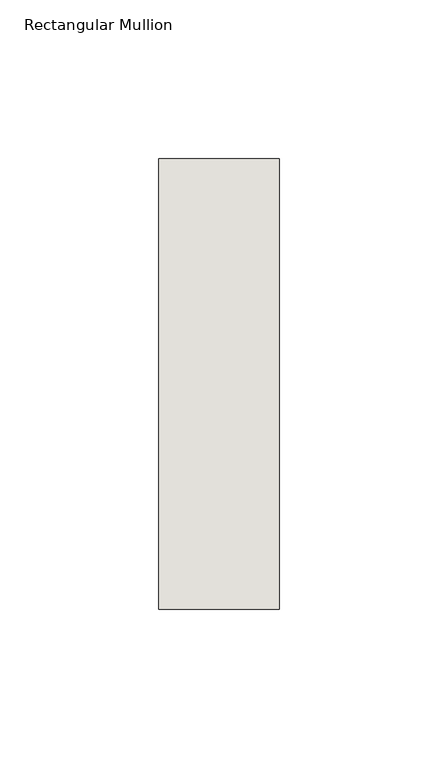
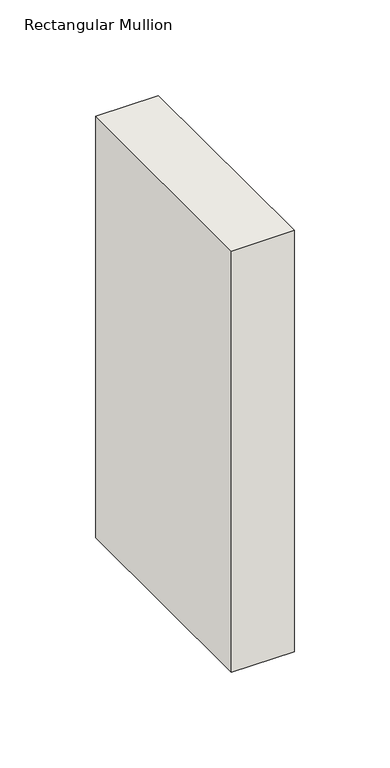
"""IFC4 building model written with IfcOpenShell, lengths in millimetres: wall geometry, Rectangular Mullion : NLRS_21_CWM_hsb-regel 38x142_gen_rsf."""

from ifc_helpers import new_model, si_unit, frame, origin, place, context, project, spatial, polyline, outline, extrude, source, transform, mapped, element, save


def rectangular_mullion_985b883b(model_context):
    return source(origin(), model_context, "Body", "SweptSolid", [
        extrude(outline(polyline([(-38.0, -71.0), (-38.0, 71.0), (0.0, 71.0), (0.0, -71.0), (-38.0, -71.0)])), frame((0.0, 0.0, -269.0000003), z_axis=(0.0, 0.0, 1.0), x_axis=(1.0, 0.0, 0.0)), (0.0, 0.0, 1.0), 269.0000003),
    ])


if __name__ == "__main__":
    model = new_model("IFC4")
    model_context = context("Model", 3, world=origin())
    ifc_project = project(units=[si_unit("LENGTHUNIT", "METRE", prefix="MILLI")], contexts=[model_context])
    site = spatial("IfcSite", under=ifc_project)
    building = spatial("IfcBuilding", under=site)
    placement = place(None, origin())
    rectangular_mullion_shape = rectangular_mullion_985b883b(model_context)
    element("IfcWall", 1, ObjectType="Rectangular Mullion : NLRS_21_CWM_hsb-regel 38x142_gen_rsf", at=placement, inside=building, context=model_context, shape_type="MappedRepresentation", body=[
        mapped(rectangular_mullion_shape, transform((0.0, 0.0, 0.0), x_axis=(1.0, 0.0, 0.0), y_axis=(0.0, 1.0, 0.0), z_axis=(0.0, 0.0, 1.0))),
    ])
    save(model, "model.ifc")

# Revit data of these elements
# Type "Rectangular Mullion : NLRS_21_CWM_hsb-regel 38x142_gen_rsf"
#   Type IfcGUID = "07M7mRoiH1CR8m_RSKIwpF"
#   Assembly Code = "21.10"
#   IfcExportAs = "IfcWall"
#   built-in parameter 1007322 = 0.465879 (stored number, unit not read)
#   built-in parameter 1007321 = 0.062336 (stored number, unit not read)
#   built-in parameter 1007320 = 0.062336 (stored number, unit not read)
# Element 1 (IfcWall, "Rectangular Mullion : NLRS_21_CWM_hsb-regel 38x142_gen_rsf")
#   Materials on its faces: "NLRS_i2_hout naaldhout vuren_gen_rsf"
# Materials
#   "NLRS_i2_hout naaldhout vuren_gen_rsf": class "I - Hout", colour RGB 234 199 147, transparency 0, Keynote = "i2", Manufacturer = "Revit Standards Foundation", URL = "www.revitstandards.org", Description = "hout vuren", Cost = 0
